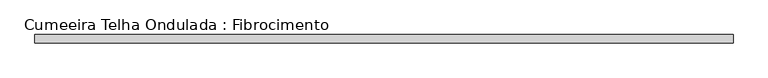
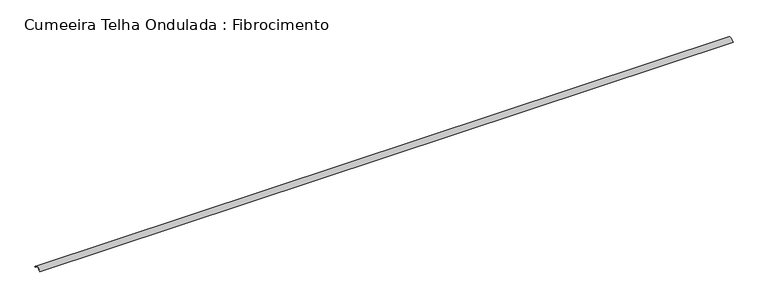
"""IFC4 building model written with IfcOpenShell, lengths in millimetres: beam geometry, Cumeeira Telha Ondulada : Fibrocimento."""

import ifcopenshell
import ifcopenshell.guid

model = None  # the IFC model being written
_history = None  # IfcOwnerHistory: only IFC2X3 demands one
_inside = {}  # id of a spatial element -> (the spatial element, [elements in it])
_under = {}  # id of a project, library or spatial element -> (it, [spatial elements below it])
_declared = {}  # id of a project -> (the project, [libraries it declares])
_typed = {}  # id of a type object -> (the type object, [elements of that type])
_made_of = {}  # id of a material, layer set ... -> (it, [elements and type objects made of it])


def new_model(schema):
    """Start an empty IFC model of exactly this schema.

    Asked for "IFC4X3", IfcOpenShell would pick the latest addendum, in which some entities
    have other attributes; the version numbers below select the first issue.
    IFC2X3 requires an IfcOwnerHistory on every rooted entity: one is made here for all.
    """
    global model, _history
    if schema == "IFC4X3":
        model = ifcopenshell.file(schema_version=(4, 3, 0, 0))
    else:
        model = ifcopenshell.file(schema=schema)
    _inside.clear()
    _under.clear()
    _declared.clear()
    _typed.clear()
    _made_of.clear()
    _history = None
    if model.schema == "IFC2X3":
        org = make("IfcOrganization", Name="unknown")
        user = make(
            "IfcPersonAndOrganization",
            ThePerson=make("IfcPerson", FamilyName="unknown"),
            TheOrganization=org,
        )
        app = make(
            "IfcApplication",
            ApplicationDeveloper=org,
            Version="unknown",
            ApplicationFullName="unknown",
            ApplicationIdentifier="unknown",
        )
        _history = make(
            "IfcOwnerHistory",
            OwningUser=user,
            OwningApplication=app,
            ChangeAction="ADDED",
            CreationDate=0,
        )
    return model


def make(cls, **values):
    """One entity of the class cls with the attributes given. An attribute that is None is left unset."""
    return model.create_entity(
        cls, **{name: value for name, value in values.items() if value is not None}
    )


def rooted(cls, **values):
    """An entity with a GlobalId (a new one), such as an element, a storey or a relation."""
    return make(cls, GlobalId=ifcopenshell.guid.new(), OwnerHistory=_history, **values)


def si_unit(unit_type, name, prefix=None):
    """IfcSIUnit, for example si_unit("LENGTHUNIT", "METRE", prefix="MILLI")."""
    return make("IfcSIUnit", UnitType=unit_type, Prefix=prefix, Name=name)


def assignment(units):
    """IfcUnitAssignment: the units of a project."""
    return None if units is None else make("IfcUnitAssignment", Units=units)


def point(xyz):
    """IfcCartesianPoint."""
    return None if xyz is None else make("IfcCartesianPoint", Coordinates=xyz)


def direction(xyz):
    """IfcDirection."""
    return None if xyz is None else make("IfcDirection", DirectionRatios=xyz)


def frame(location, z_axis=None, x_axis=None):
    """IfcAxis2Placement3D, a coordinate frame: its origin and axes. An axis left out is left unset."""
    return make(
        "IfcAxis2Placement3D",
        Location=point(location),
        Axis=direction(z_axis),
        RefDirection=direction(x_axis),
    )


def frame_2d(location, x_axis=None):
    """IfcAxis2Placement2D, a coordinate frame in the plane: its origin and x axis."""
    return make(
        "IfcAxis2Placement2D", Location=point(location), RefDirection=direction(x_axis)
    )


def origin():
    """The frame at (0, 0, 0) with its axes left unset."""
    return frame((0.0, 0.0, 0.0))


def place(relative_to, where):
    """IfcLocalPlacement: puts the frame where relative to a parent placement (None: the world)."""
    return make(
        "IfcLocalPlacement", PlacementRelTo=relative_to, RelativePlacement=where
    )


def context(
    kind, dimensions, precision=None, world=None, true_north=None, identifier=None
):
    """IfcGeometricRepresentationContext, for example the 3D "Model" context."""
    return make(
        "IfcGeometricRepresentationContext",
        ContextIdentifier=identifier,
        ContextType=kind,
        CoordinateSpaceDimension=dimensions,
        Precision=precision,
        WorldCoordinateSystem=world,
        TrueNorth=true_north,
    )


def project(units=None, contexts=None):
    """IfcProject with its units and contexts."""
    return rooted(
        "IfcProject",
        Name="project",
        RepresentationContexts=contexts,
        UnitsInContext=assignment(units),
    )


def spatial(cls, under=None, at=None, **own):
    """A site, building, storey or space (cls), placed at a placement, below another one or the project."""
    s = rooted(cls, ObjectPlacement=at, **own)
    if under is not None:
        _under.setdefault(under.id(), (under, []))[1].append(s)
    return s


def polyline(points):
    """IfcPolyline through the points."""
    return make("IfcPolyline", Points=[point(p) for p in points])


def circle_curve(where, radius):
    """IfcCircle in the frame where."""
    return make("IfcCircle", Position=where, Radius=radius)


def trimmed(basis, trim1, trim2, sense, master):
    """IfcTrimmedCurve: the piece of a basis curve between two trims."""
    return make(
        "IfcTrimmedCurve",
        BasisCurve=basis,
        Trim1=trim1,
        Trim2=trim2,
        SenseAgreement=sense,
        MasterRepresentation=master,
    )


def segment(curve, same_sense, transition):
    """IfcCompositeCurveSegment."""
    return make(
        "IfcCompositeCurveSegment",
        Transition=transition,
        SameSense=same_sense,
        ParentCurve=curve,
    )


def composite_curve(segments, self_intersect=None):
    """IfcCompositeCurve: segments joined end to end."""
    return make("IfcCompositeCurve", Segments=segments, SelfIntersect=self_intersect)


def outline(outer, holes=None, kind="AREA"):
    """IfcArbitraryClosedProfileDef: a profile drawn as a closed curve; with holes, ...WithVoids."""
    if holes is None:
        return make("IfcArbitraryClosedProfileDef", ProfileType=kind, OuterCurve=outer)
    return make(
        "IfcArbitraryProfileDefWithVoids",
        ProfileType=kind,
        OuterCurve=outer,
        InnerCurves=holes,
    )


def extrude(swept, where, along, depth):
    """IfcExtrudedAreaSolid: the profile swept, set in the frame where, extruded along a direction by depth."""
    return make(
        "IfcExtrudedAreaSolid",
        SweptArea=swept,
        Position=where,
        ExtrudedDirection=direction(along),
        Depth=depth,
    )


def shape(context_of_items, identifier, shape_type, items):
    """IfcShapeRepresentation: the items that make up one representation, for example the "Body"."""
    return make(
        "IfcShapeRepresentation",
        ContextOfItems=context_of_items,
        RepresentationIdentifier=identifier,
        RepresentationType=shape_type,
        Items=items,
    )


def source(mapping_origin, context_of_items, identifier, shape_type, items):
    """IfcRepresentationMap: a shape defined once, which mapped items show again and again."""
    return make(
        "IfcRepresentationMap",
        MappingOrigin=mapping_origin,
        MappedRepresentation=shape(context_of_items, identifier, shape_type, items),
    )


def transform(
    local_origin,
    x_axis=None,
    y_axis=None,
    z_axis=None,
    scale=None,
    scale2=None,
    scale3=None,
    uniform=True,
):
    """IfcCartesianTransformationOperator3D, or its non-uniform kind. x_axis, y_axis, z_axis: its Axis1, 2, 3."""
    if uniform:
        return make(
            "IfcCartesianTransformationOperator3D",
            Axis1=direction(x_axis),
            Axis2=direction(y_axis),
            LocalOrigin=point(local_origin),
            Scale=scale,
            Axis3=direction(z_axis),
        )
    return make(
        "IfcCartesianTransformationOperator3DnonUniform",
        Axis1=direction(x_axis),
        Axis2=direction(y_axis),
        LocalOrigin=point(local_origin),
        Scale=scale,
        Axis3=direction(z_axis),
        Scale2=scale2,
        Scale3=scale3,
    )


def mapped(mapping_source, mapping_target):
    """IfcMappedItem: shows the shape of a source again, moved by a transform."""
    return make(
        "IfcMappedItem", MappingSource=mapping_source, MappingTarget=mapping_target
    )


def made_of(thing, what):
    """Note that an element or type object is made of a material, layer set ...; save() writes the relation."""
    if what is not None:
        _made_of.setdefault(what.id(), (what, []))[1].append(thing)
    return thing


def element(
    cls,
    number,
    at=None,
    inside=None,
    cuts=None,
    type_object=None,
    material=None,
    context=None,
    identifier="Body",
    shape_type=None,
    held_by="IfcProductDefinitionShape",
    body=None,
    shapes=None,
    **own,
):
    """One element of the class cls, such as IfcWall. Its Tag is "e" and its number.

    at: its placement. inside: the storey or other place that contains it. cuts: it is an
    opening in that element (IfcRelVoidsElement). A single representation is given by context,
    identifier, shape_type and body (its items); several are given by shapes. held_by: the class
    of the entity that holds the representations. save() writes the other relations.
    """
    e = rooted(cls, Tag="e%d" % number, ObjectPlacement=at, **own)
    if body is not None:
        shapes = [shape(context, identifier, shape_type, body)]
    if shapes is not None:
        e.Representation = make(held_by, Representations=shapes)
    if inside is not None:
        _inside.setdefault(inside.id(), (inside, []))[1].append(e)
    if cuts is not None:
        rooted(
            "IfcRelVoidsElement", RelatingBuildingElement=cuts, RelatedOpeningElement=e
        )
    if type_object is not None:
        _typed.setdefault(type_object.id(), (type_object, []))[1].append(e)
    return made_of(e, material)


def aggregate(whole, parts):
    """IfcRelAggregates: a whole, such as a stair, and the parts it consists of."""
    return rooted("IfcRelAggregates", RelatingObject=whole, RelatedObjects=parts)


def save(model, path):
    """Write the relations noted so far, then the file.

    IfcRelAggregates (storeys below a building ...), IfcRelContainedInSpatialStructure (elements
    in a storey), IfcRelDefinesByType, IfcRelAssociatesMaterial and IfcRelDeclares: one each for
    every whole, place, type object, material and project.
    """
    for whole, parts in _under.values():
        aggregate(whole, parts)
    for where, things in _inside.values():
        rooted(
            "IfcRelContainedInSpatialStructure",
            RelatedElements=things,
            RelatingStructure=where,
        )
    for kind, things in _typed.values():
        rooted("IfcRelDefinesByType", RelatedObjects=things, RelatingType=kind)
    for what, things in _made_of.values():
        rooted("IfcRelAssociatesMaterial", RelatedObjects=things, RelatingMaterial=what)
    for by, libraries in _declared.values():
        rooted("IfcRelDeclares", RelatingContext=by, RelatedDefinitions=libraries)
    model.write(path)


def cumeeira_telha_ondulada_fibrocimento_c9eafb3e(model_context):
    return source(origin(), model_context, "Body", "SweptSolid", [
        extrude(outline(composite_curve([segment(polyline([(58.3970135, 42.4437972), (53.9055884, 40.2467307)]), True, "CONTINUOUS"), segment(trimmed(circle_curve(frame_2d((-1.6029865, 13.0936483)), 61.7939461), [point((53.9055884, 40.2467307))], [point((-57.1115615, 40.2467307))], True, "CARTESIAN"), True, "CONTINUOUS"), segment(polyline([(-57.1115615, 40.2467307), (-61.6029865, 42.4437972)]), True, "CONTINUOUS"), segment(trimmed(circle_curve(frame_2d((-1.6029865, 13.0936483)), 66.7939461), [point((-61.6029865, 42.4437972))], [point((58.3970135, 42.4437972))], False, "CARTESIAN"), True, "CONTINUOUS")], self_intersect=False)), frame((-4969.5, 0.0, 0.0), z_axis=(1.0, 0.0, 0.0), x_axis=(0.0, 1.0, 0.0)), (0.0, 0.0, 1.0), 9939.0),
    ])


if __name__ == "__main__":
    model = new_model("IFC4")
    model_context = context("Model", 3, world=origin())
    ifc_project = project(units=[si_unit("LENGTHUNIT", "METRE", prefix="MILLI")], contexts=[model_context])
    site = spatial("IfcSite", under=ifc_project)
    building = spatial("IfcBuilding", under=site)
    placement = place(None, origin())
    cumeeira_telha_ondulada_fibrocimento_shape = cumeeira_telha_ondulada_fibrocimento_c9eafb3e(model_context)
    element("IfcBeam", 1, ObjectType="Cumeeira Telha Ondulada : Fibrocimento", at=placement, inside=building, context=model_context, shape_type="MappedRepresentation", body=[
        mapped(cumeeira_telha_ondulada_fibrocimento_shape, transform((0.0, 0.0, 0.0), x_axis=(1.0, 0.0, 0.0), y_axis=(0.0, 1.0, 0.0), z_axis=(0.0, 0.0, 1.0))),
    ])
    save(model, "model.ifc")

# Revit data of these elements
# Type "Cumeeira Telha Ondulada : Fibrocimento"
#   Cost = 5
#   Length [instance default] = 1.524 m
#   b = 0.07 m
#   h = 0.16 m
#   Structural Material = .TELHA DE FIBROCIMENTO
#   Assembly Code = ""
# Element 1 (IfcBeam, "Cumeeira Telha Ondulada : Fibrocimento")
#   Materials on its faces: ".TELHA DE FIBROCIMENTO"
# Materials
#   ".TELHA DE FIBROCIMENTO": class "CC_TELHADO", colour RGB 77 77 76, transparency 0, Description = "TELHA ONDULADA FIBROCIMENTO", Cost = 0
